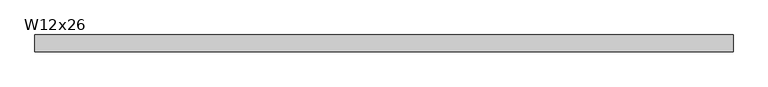
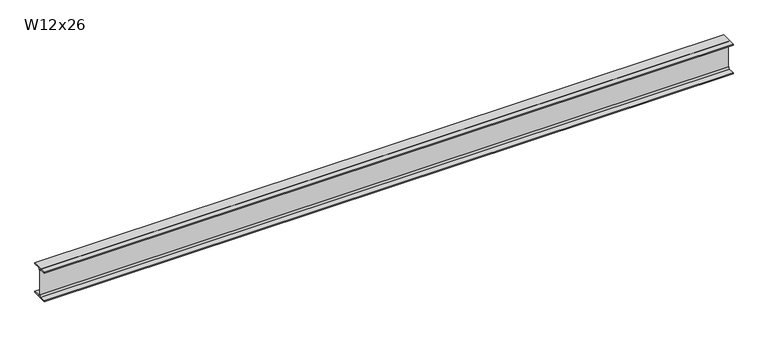
"""IFC4 building model written with IfcOpenShell, lengths in millimetres: beam geometry, RME W-Wide Flange : W12x26."""

from ifc_helpers import new_model, si_unit, point, frame, frame_2d, origin, place, context, project, spatial, polyline, circle_curve, trimmed, segment, composite_curve, outline, extrude, source, transform, mapped, element, save


def w12x26_bd1806ec(model_context):
    return source(origin(), model_context, "Body", "SweptSolid", [
        extrude(outline(composite_curve([segment(polyline([(82.423, -145.288), (82.423, -154.94), (-82.423, -154.94), (-82.423, -145.288), (-20.2565, -145.288)]), True, "CONTINUOUS"), segment(trimmed(circle_curve(frame_2d((-20.2565, -127.9525)), 17.3355), [point((-20.2565, -145.288))], [point((-2.921, -127.9525))], True, "CARTESIAN"), True, "CONTINUOUS"), segment(polyline([(-2.921, -127.9525), (-2.921, 127.9525)]), True, "CONTINUOUS"), segment(trimmed(circle_curve(frame_2d((-20.2565, 127.9525)), 17.3355), [point((-2.921, 127.9525))], [point((-20.2565, 145.288))], True, "CARTESIAN"), True, "CONTINUOUS"), segment(polyline([(-20.2565, 145.288), (-82.423, 145.288), (-82.423, 154.94), (82.423, 154.94), (82.423, 145.288), (20.2565, 145.288)]), True, "CONTINUOUS"), segment(trimmed(circle_curve(frame_2d((20.2565, 127.9525)), 17.3355), [point((20.2565, 145.288))], [point((2.921, 127.9525))], True, "CARTESIAN"), True, "CONTINUOUS"), segment(polyline([(2.921, 127.9525), (2.921, -127.9525)]), True, "CONTINUOUS"), segment(trimmed(circle_curve(frame_2d((20.2565, -127.9525)), 17.3355), [point((2.921, -127.9525))], [point((20.2565, -145.288))], True, "CARTESIAN"), True, "CONTINUOUS"), segment(polyline([(20.2565, -145.288), (82.423, -145.288)]), True, "CONTINUOUS")], self_intersect=False)), frame((-3587.75, 0.0, 0.0), z_axis=(1.0, 0.0, 0.0), x_axis=(0.0, 1.0, 0.0)), (0.0, 0.0, 1.0), 6870.7),
    ])


if __name__ == "__main__":
    model = new_model("IFC4")
    model_context = context("Model", 3, world=origin())
    ifc_project = project(units=[si_unit("LENGTHUNIT", "METRE", prefix="MILLI")], contexts=[model_context])
    site = spatial("IfcSite", under=ifc_project)
    building = spatial("IfcBuilding", under=site)
    placement = place(None, origin())
    w12x26_shape = w12x26_bd1806ec(model_context)
    element("IfcBeam", 1, ObjectType="RME W-Wide Flange : W12x26", at=placement, inside=building, context=model_context, shape_type="MappedRepresentation", body=[
        mapped(w12x26_shape, transform((0.0, 0.0, 0.0), x_axis=(1.0, 0.0, 0.0), y_axis=(0.0, 1.0, 0.0), z_axis=(0.0, 0.0, 1.0))),
    ])
    save(model, "model.ifc")

# Revit data of these elements
# Type "RME W-Wide Flange : W12x26"
#   WELD P [instance default] = ""
#   WELD LE [instance default] = ""
#   WELD D [instance default] = ""
#   TOP SECTION SIZE [instance default] = ""
#   TOP SECTION LENGTH [instance default] = ""
#   REMARKS [instance default] = ""
#   REINF TYPE [instance default] = ""
#   Nominal Size = "W24"
#   End Bearing Capacity [instance default] = ""
#   BOT SECTION SIZE [instance default] = ""
#   BOT SECTION LENGTH [instance default] = ""
#   Assembly Code = "B10"
#   W = 26
#   Start Extension Calculation [instance default] = 10' - 0"
#   Start Extension [instance default] = -0' - 0 1/2"
#   End Extension Calculation [instance default] = 10' - 0"
#   End Extension [instance default] = -0' - 0 1/2"
#   Length [instance default] = 5' - 0"
#   bf = 0' - 6.49"
#   d = 1' - 0.2"
#   k = 0' - 1 1/16"
#   k2 = 0' - 0.6825"
#   tf = 0' - 0.38"
#   tw = 0' - 0.23"
#   A = 0.053125 SF
#   Structural Material [instance default] = Metal - Steel - ASTM A992
# Element 1 (IfcBeam, "RME W-Wide Flange : W12x26")
#   Length = 23' - 6 1/2"
#   Materials on its faces: "Metal - Steel - ASTM A992"
# Materials
#   "Metal - Steel - ASTM A992": class "Metal", colour RGB 255 128 0, transparency 0
